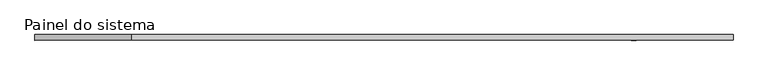
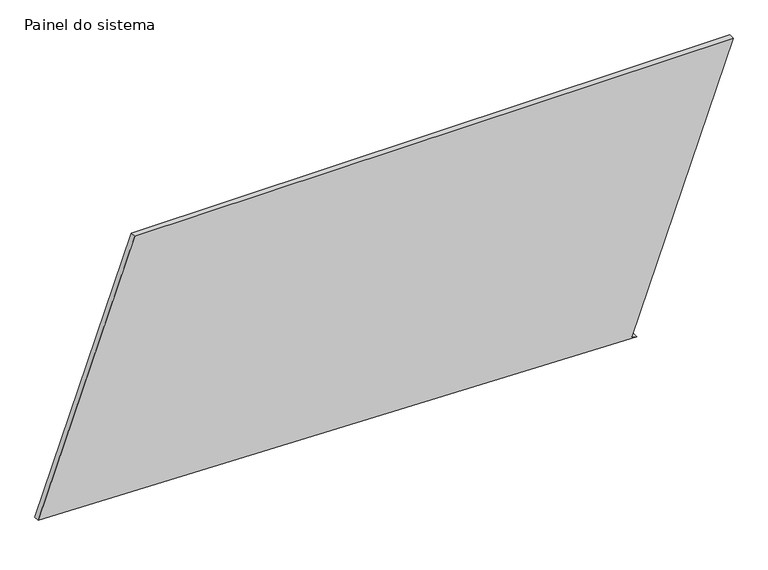
"""IFC4 building model written with IfcOpenShell, lengths in millimetres: plate geometry, Painel do sistema : Envidraçado."""

from ifc_helpers import new_model, si_unit, frame, origin, place, context, project, spatial, polyline, outline, extrude, source, transform, mapped, element, save


def painel_do_sistema_e17ca7a4(model_context):
    return source(origin(), model_context, "Body", "SweptSolid", [
        extrude(outline(polyline([(0.0, 1137.6221355), (8.505028, 1114.113318), (1276.6450236, 1572.9014382), (1276.6450236, -1136.3255962), (69.9021678, -1572.9014382), (0.0, 1137.6221355)])), frame((0.0, 24.5, 0.0), z_axis=(0.0, 1.0, 0.0), x_axis=(0.0, 0.0, 1.0)), (0.0, 0.0, 1.0), 25.0),
    ])


if __name__ == "__main__":
    model = new_model("IFC4")
    model_context = context("Model", 3, world=origin())
    ifc_project = project(units=[si_unit("LENGTHUNIT", "METRE", prefix="MILLI")], contexts=[model_context])
    site = spatial("IfcSite", under=ifc_project)
    building = spatial("IfcBuilding", under=site)
    placement = place(None, origin())
    painel_do_sistema_shape = painel_do_sistema_e17ca7a4(model_context)
    element("IfcPlate", 1, ObjectType="Painel do sistema : Envidraçado", at=placement, inside=building, context=model_context, shape_type="MappedRepresentation", body=[
        mapped(painel_do_sistema_shape, transform((0.0, 0.0, 0.0), x_axis=(1.0, 0.0, 0.0), y_axis=(0.0, 1.0, 0.0), z_axis=(0.0, 0.0, 1.0))),
    ])
    save(model, "model.ifc")

# Revit data of these elements
# Type "Painel do sistema : Envidraçado"
#   Construction Type Id = "GSP4R"
#   Analytic Construction = "Vidraça única Pilkington 1/8 pol"
#   Visual Light Transmittance = 0.9
#   Solar Heat Gain Coefficient = 0.86
#   Heat Transfer Coefficient (U) = 6.7069 W/(m²·K)
# Element 1 (IfcPlate, "Painel do sistema : Envidraçado")
#   Materials on its faces: "Vidro"
# Materials
#   "Vidro": class "Vidro", colour RGB 0 128 192, transparency 0.9, Description = "Vidro de sílica", Cost = 0
